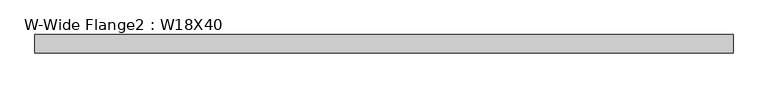
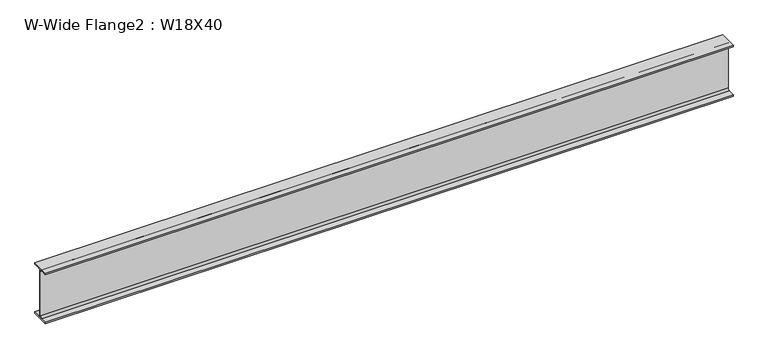
"""IFC4 building model written with IfcOpenShell, lengths in millimetres: beam geometry, W-Wide Flange2 : W18X40."""

from ifc_helpers import new_model, si_unit, point, frame, frame_2d, origin, place, context, project, spatial, polyline, circle_curve, trimmed, segment, composite_curve, outline, extrude, source, transform, mapped, element, save


def w_wide_flange2_w18x40_2cba9d45(model_context):
    return source(origin(), model_context, "Body", "SweptSolid", [
        extrude(outline(composite_curve([segment(polyline([(76.454, -213.995), (76.454, -227.33), (-76.454, -227.33), (-76.454, -213.995), (-20.828, -213.995)]), True, "CONTINUOUS"), segment(trimmed(circle_curve(frame_2d((-20.828, -197.1675)), 16.8275), [point((-20.828, -213.995))], [point((-4.0005, -197.1675))], True, "CARTESIAN"), True, "CONTINUOUS"), segment(polyline([(-4.0005, -197.1675), (-4.0005, 197.1675)]), True, "CONTINUOUS"), segment(trimmed(circle_curve(frame_2d((-20.828, 197.1675)), 16.8275), [point((-4.0005, 197.1675))], [point((-20.828, 213.995))], True, "CARTESIAN"), True, "CONTINUOUS"), segment(polyline([(-20.828, 213.995), (-76.454, 213.995), (-76.454, 227.33), (76.454, 227.33), (76.454, 213.995), (20.828, 213.995)]), True, "CONTINUOUS"), segment(trimmed(circle_curve(frame_2d((20.828, 197.1675)), 16.8275), [point((20.828, 213.995))], [point((4.0005, 197.1675))], True, "CARTESIAN"), True, "CONTINUOUS"), segment(polyline([(4.0005, 197.1675), (4.0005, -197.1675)]), True, "CONTINUOUS"), segment(trimmed(circle_curve(frame_2d((20.828, -197.1675)), 16.8275), [point((4.0005, -197.1675))], [point((20.828, -213.995))], True, "CARTESIAN"), True, "CONTINUOUS"), segment(polyline([(20.828, -213.995), (76.454, -213.995)]), True, "CONTINUOUS")], self_intersect=False)), frame((-2883.69375, 0.0, 0.0), z_axis=(1.0, 0.0, 0.0), x_axis=(0.0, 1.0, 0.0)), (0.0, 0.0, 1.0), 5824.5375),
    ])


if __name__ == "__main__":
    model = new_model("IFC4")
    model_context = context("Model", 3, world=origin())
    ifc_project = project(units=[si_unit("LENGTHUNIT", "METRE", prefix="MILLI")], contexts=[model_context])
    site = spatial("IfcSite", under=ifc_project)
    building = spatial("IfcBuilding", under=site)
    placement = place(None, origin())
    w_wide_flange2_w18x40_shape = w_wide_flange2_w18x40_2cba9d45(model_context)
    element("IfcBeam", 1, ObjectType="W-Wide Flange2 : W18X40", at=placement, inside=building, context=model_context, shape_type="MappedRepresentation", body=[
        mapped(w_wide_flange2_w18x40_shape, transform((0.0, 0.0, 0.0), x_axis=(1.0, 0.0, 0.0), y_axis=(0.0, 1.0, 0.0), z_axis=(0.0, 0.0, 1.0))),
    ])
    save(model, "model.ifc")

# Revit data of these elements
# Type "W-Wide Flange2 : W18X40"
#   Assembly Code = "B10"
#   W = 40
#   Length [instance default] = 5' - 0"
#   bf = 0' - 6.02"
#   d = 1' - 5.9"
#   k = 0' - 1 3/16"
#   k2 = 0' - 0.6625"
#   tf = 0' - 0.525"
#   tw = 0' - 0.315"
#   A = 0.0819444 SF
#   Structural Material [instance default] = Steel ASTM A992
# Element 1 (IfcBeam, "W-Wide Flange2 : W18X40")
#   Materials on its faces: "Steel ASTM A992"
# Materials
#   "Steel ASTM A992": class "Metal", colour RGB 199 199 199, transparency 0, Description = "Structural steel 50ksi", Cost = 0
